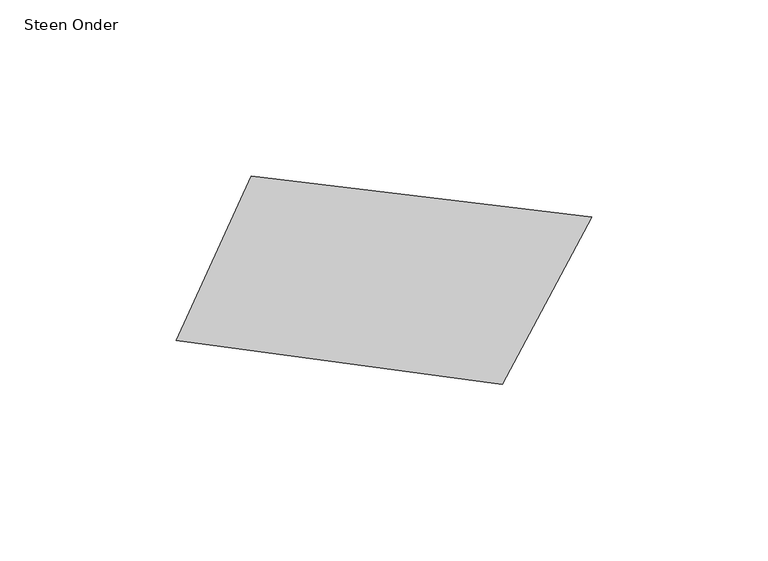
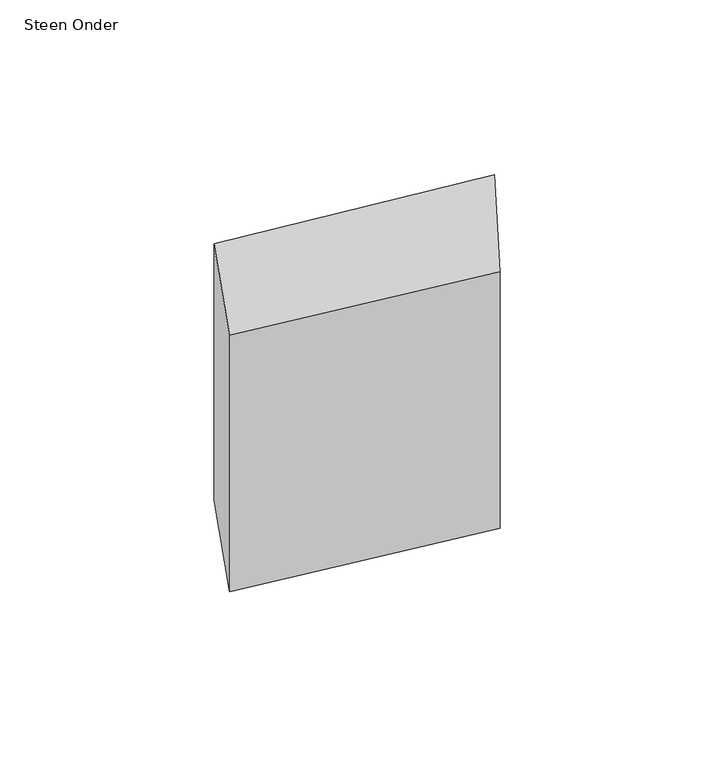
"""IFC4 building model written with IfcOpenShell, lengths in millimetres: proxy geometry, 00_GMA_steen_versie_4 : Steen Onder."""

from ifc_helpers import new_model, si_unit, frame, origin, place, context, project, spatial, polyline, outline, extrude, source, transform, mapped, element, save


def steen_onder_df57c089(model_context):
    return source(origin(), model_context, "Body", "SweptSolid", [
        extrude(outline(polyline([(149.2591289, 58.5631182), (123.7987483, 11.0079353), (31.2999852, 23.5462122), (52.5448074, 70.2334053), (149.2591289, 58.5631182)])), frame((0.0, 0.0, -100.0), z_axis=(0.0, 0.0, 1.0), x_axis=(1.0, 0.0, 0.0)), (0.0, 0.0, 1.0), 100.0),
    ])


if __name__ == "__main__":
    model = new_model("IFC4")
    model_context = context("Model", 3, world=origin())
    ifc_project = project(units=[si_unit("LENGTHUNIT", "METRE", prefix="MILLI")], contexts=[model_context])
    site = spatial("IfcSite", under=ifc_project)
    building = spatial("IfcBuilding", under=site)
    placement = place(None, origin())
    steen_onder_shape = steen_onder_df57c089(model_context)
    element("IfcBuildingElementProxy", 1, Name="00_GMA_steen_versie_4 : Steen Onder", ObjectType="00_GMA_steen_versie_4 : Steen Onder", at=placement, inside=building, context=model_context, shape_type="MappedRepresentation", body=[
        mapped(steen_onder_shape, transform((0.0, 0.0, 0.0), x_axis=(1.0, 0.0, 0.0), y_axis=(0.0, 1.0, 0.0), z_axis=(0.0, 0.0, 1.0))),
    ])
    save(model, "model.ifc")

# Revit data of these elements
# Type "00_GMA_steen_versie_4 : Steen Onder"
#   StootVoegHalfBoven [instance default] = 5 mm
#   StootVoegHalf [instance default] = 5 mm
#   StootVoegBreedteOnder = 10 mm
#   StootVoegBreedteBoven = 10 mm
#   Steendikte = 100 mm
#   LintVoegOnderHalf = 0 mm
#   LintVoegOnder = 0 mm
#   LintVoegBovenHalf = 5 mm
#   LintVoegBoven = 10 mm
#   materiaal = none
#   MateriaalVoeg = none
#   Default Elevation = 0
